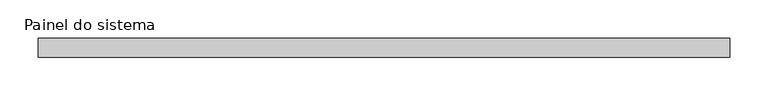
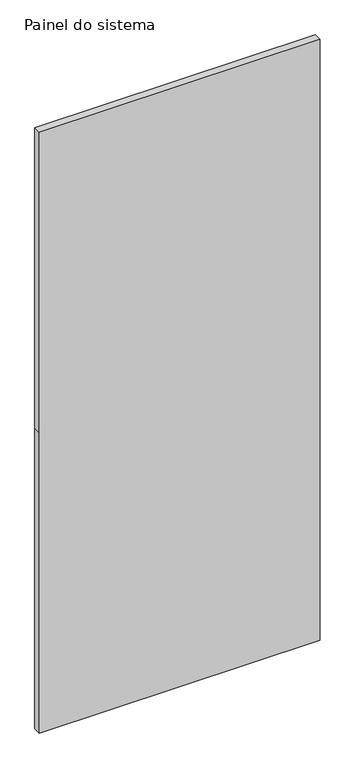
"""IFC4 building model written with IfcOpenShell, lengths in millimetres: plate geometry, Painel do sistema : Envidraçado."""

import ifcopenshell
import ifcopenshell.guid

model = None  # the IFC model being written
_history = None  # IfcOwnerHistory: only IFC2X3 demands one
_inside = {}  # id of a spatial element -> (the spatial element, [elements in it])
_under = {}  # id of a project, library or spatial element -> (it, [spatial elements below it])
_declared = {}  # id of a project -> (the project, [libraries it declares])
_typed = {}  # id of a type object -> (the type object, [elements of that type])
_made_of = {}  # id of a material, layer set ... -> (it, [elements and type objects made of it])


def new_model(schema):
    """Start an empty IFC model of exactly this schema.

    Asked for "IFC4X3", IfcOpenShell would pick the latest addendum, in which some entities
    have other attributes; the version numbers below select the first issue.
    IFC2X3 requires an IfcOwnerHistory on every rooted entity: one is made here for all.
    """
    global model, _history
    if schema == "IFC4X3":
        model = ifcopenshell.file(schema_version=(4, 3, 0, 0))
    else:
        model = ifcopenshell.file(schema=schema)
    _inside.clear()
    _under.clear()
    _declared.clear()
    _typed.clear()
    _made_of.clear()
    _history = None
    if model.schema == "IFC2X3":
        org = make("IfcOrganization", Name="unknown")
        user = make(
            "IfcPersonAndOrganization",
            ThePerson=make("IfcPerson", FamilyName="unknown"),
            TheOrganization=org,
        )
        app = make(
            "IfcApplication",
            ApplicationDeveloper=org,
            Version="unknown",
            ApplicationFullName="unknown",
            ApplicationIdentifier="unknown",
        )
        _history = make(
            "IfcOwnerHistory",
            OwningUser=user,
            OwningApplication=app,
            ChangeAction="ADDED",
            CreationDate=0,
        )
    return model


def make(cls, **values):
    """One entity of the class cls with the attributes given. An attribute that is None is left unset."""
    return model.create_entity(
        cls, **{name: value for name, value in values.items() if value is not None}
    )


def rooted(cls, **values):
    """An entity with a GlobalId (a new one), such as an element, a storey or a relation."""
    return make(cls, GlobalId=ifcopenshell.guid.new(), OwnerHistory=_history, **values)


def si_unit(unit_type, name, prefix=None):
    """IfcSIUnit, for example si_unit("LENGTHUNIT", "METRE", prefix="MILLI")."""
    return make("IfcSIUnit", UnitType=unit_type, Prefix=prefix, Name=name)


def assignment(units):
    """IfcUnitAssignment: the units of a project."""
    return None if units is None else make("IfcUnitAssignment", Units=units)


def point(xyz):
    """IfcCartesianPoint."""
    return None if xyz is None else make("IfcCartesianPoint", Coordinates=xyz)


def direction(xyz):
    """IfcDirection."""
    return None if xyz is None else make("IfcDirection", DirectionRatios=xyz)


def frame(location, z_axis=None, x_axis=None):
    """IfcAxis2Placement3D, a coordinate frame: its origin and axes. An axis left out is left unset."""
    return make(
        "IfcAxis2Placement3D",
        Location=point(location),
        Axis=direction(z_axis),
        RefDirection=direction(x_axis),
    )


def origin():
    """The frame at (0, 0, 0) with its axes left unset."""
    return frame((0.0, 0.0, 0.0))


def place(relative_to, where):
    """IfcLocalPlacement: puts the frame where relative to a parent placement (None: the world)."""
    return make(
        "IfcLocalPlacement", PlacementRelTo=relative_to, RelativePlacement=where
    )


def context(
    kind, dimensions, precision=None, world=None, true_north=None, identifier=None
):
    """IfcGeometricRepresentationContext, for example the 3D "Model" context."""
    return make(
        "IfcGeometricRepresentationContext",
        ContextIdentifier=identifier,
        ContextType=kind,
        CoordinateSpaceDimension=dimensions,
        Precision=precision,
        WorldCoordinateSystem=world,
        TrueNorth=true_north,
    )


def project(units=None, contexts=None):
    """IfcProject with its units and contexts."""
    return rooted(
        "IfcProject",
        Name="project",
        RepresentationContexts=contexts,
        UnitsInContext=assignment(units),
    )


def spatial(cls, under=None, at=None, **own):
    """A site, building, storey or space (cls), placed at a placement, below another one or the project."""
    s = rooted(cls, ObjectPlacement=at, **own)
    if under is not None:
        _under.setdefault(under.id(), (under, []))[1].append(s)
    return s


def polyline(points):
    """IfcPolyline through the points."""
    return make("IfcPolyline", Points=[point(p) for p in points])


def outline(outer, holes=None, kind="AREA"):
    """IfcArbitraryClosedProfileDef: a profile drawn as a closed curve; with holes, ...WithVoids."""
    if holes is None:
        return make("IfcArbitraryClosedProfileDef", ProfileType=kind, OuterCurve=outer)
    return make(
        "IfcArbitraryProfileDefWithVoids",
        ProfileType=kind,
        OuterCurve=outer,
        InnerCurves=holes,
    )


def extrude(swept, where, along, depth):
    """IfcExtrudedAreaSolid: the profile swept, set in the frame where, extruded along a direction by depth."""
    return make(
        "IfcExtrudedAreaSolid",
        SweptArea=swept,
        Position=where,
        ExtrudedDirection=direction(along),
        Depth=depth,
    )


def shape(context_of_items, identifier, shape_type, items):
    """IfcShapeRepresentation: the items that make up one representation, for example the "Body"."""
    return make(
        "IfcShapeRepresentation",
        ContextOfItems=context_of_items,
        RepresentationIdentifier=identifier,
        RepresentationType=shape_type,
        Items=items,
    )


def source(mapping_origin, context_of_items, identifier, shape_type, items):
    """IfcRepresentationMap: a shape defined once, which mapped items show again and again."""
    return make(
        "IfcRepresentationMap",
        MappingOrigin=mapping_origin,
        MappedRepresentation=shape(context_of_items, identifier, shape_type, items),
    )


def transform(
    local_origin,
    x_axis=None,
    y_axis=None,
    z_axis=None,
    scale=None,
    scale2=None,
    scale3=None,
    uniform=True,
):
    """IfcCartesianTransformationOperator3D, or its non-uniform kind. x_axis, y_axis, z_axis: its Axis1, 2, 3."""
    if uniform:
        return make(
            "IfcCartesianTransformationOperator3D",
            Axis1=direction(x_axis),
            Axis2=direction(y_axis),
            LocalOrigin=point(local_origin),
            Scale=scale,
            Axis3=direction(z_axis),
        )
    return make(
        "IfcCartesianTransformationOperator3DnonUniform",
        Axis1=direction(x_axis),
        Axis2=direction(y_axis),
        LocalOrigin=point(local_origin),
        Scale=scale,
        Axis3=direction(z_axis),
        Scale2=scale2,
        Scale3=scale3,
    )


def mapped(mapping_source, mapping_target):
    """IfcMappedItem: shows the shape of a source again, moved by a transform."""
    return make(
        "IfcMappedItem", MappingSource=mapping_source, MappingTarget=mapping_target
    )


def made_of(thing, what):
    """Note that an element or type object is made of a material, layer set ...; save() writes the relation."""
    if what is not None:
        _made_of.setdefault(what.id(), (what, []))[1].append(thing)
    return thing


def element(
    cls,
    number,
    at=None,
    inside=None,
    cuts=None,
    type_object=None,
    material=None,
    context=None,
    identifier="Body",
    shape_type=None,
    held_by="IfcProductDefinitionShape",
    body=None,
    shapes=None,
    **own,
):
    """One element of the class cls, such as IfcWall. Its Tag is "e" and its number.

    at: its placement. inside: the storey or other place that contains it. cuts: it is an
    opening in that element (IfcRelVoidsElement). A single representation is given by context,
    identifier, shape_type and body (its items); several are given by shapes. held_by: the class
    of the entity that holds the representations. save() writes the other relations.
    """
    e = rooted(cls, Tag="e%d" % number, ObjectPlacement=at, **own)
    if body is not None:
        shapes = [shape(context, identifier, shape_type, body)]
    if shapes is not None:
        e.Representation = make(held_by, Representations=shapes)
    if inside is not None:
        _inside.setdefault(inside.id(), (inside, []))[1].append(e)
    if cuts is not None:
        rooted(
            "IfcRelVoidsElement", RelatingBuildingElement=cuts, RelatedOpeningElement=e
        )
    if type_object is not None:
        _typed.setdefault(type_object.id(), (type_object, []))[1].append(e)
    return made_of(e, material)


def aggregate(whole, parts):
    """IfcRelAggregates: a whole, such as a stair, and the parts it consists of."""
    return rooted("IfcRelAggregates", RelatingObject=whole, RelatedObjects=parts)


def save(model, path):
    """Write the relations noted so far, then the file.

    IfcRelAggregates (storeys below a building ...), IfcRelContainedInSpatialStructure (elements
    in a storey), IfcRelDefinesByType, IfcRelAssociatesMaterial and IfcRelDeclares: one each for
    every whole, place, type object, material and project.
    """
    for whole, parts in _under.values():
        aggregate(whole, parts)
    for where, things in _inside.values():
        rooted(
            "IfcRelContainedInSpatialStructure",
            RelatedElements=things,
            RelatingStructure=where,
        )
    for kind, things in _typed.values():
        rooted("IfcRelDefinesByType", RelatedObjects=things, RelatingType=kind)
    for what, things in _made_of.values():
        rooted("IfcRelAssociatesMaterial", RelatedObjects=things, RelatingMaterial=what)
    for by, libraries in _declared.values():
        rooted("IfcRelDeclares", RelatingContext=by, RelatedDefinitions=libraries)
    model.write(path)


def painel_do_sistema_78d5b6fe(model_context):
    return source(origin(), model_context, "Body", "SweptSolid", [
        extrude(outline(polyline([(0.0, -453.0083333), (0.0, 453.0083333), (1025.0, 453.0083333), (2050.0, 453.0083333), (2050.0, -453.0083333), (1025.0, -453.0083333), (0.0, -453.0083333)])), frame((0.0, 24.5, 0.0), z_axis=(0.0, 1.0, 0.0), x_axis=(0.0, 0.0, 1.0)), (0.0, 0.0, 1.0), 25.0),
    ])


if __name__ == "__main__":
    model = new_model("IFC4")
    model_context = context("Model", 3, world=origin())
    ifc_project = project(units=[si_unit("LENGTHUNIT", "METRE", prefix="MILLI")], contexts=[model_context])
    site = spatial("IfcSite", under=ifc_project)
    building = spatial("IfcBuilding", under=site)
    placement = place(None, origin())
    painel_do_sistema_shape = painel_do_sistema_78d5b6fe(model_context)
    element("IfcPlate", 1, ObjectType="Painel do sistema : Envidraçado", at=placement, inside=building, context=model_context, shape_type="MappedRepresentation", body=[
        mapped(painel_do_sistema_shape, transform((0.0, 0.0, 0.0), x_axis=(1.0, 0.0, 0.0), y_axis=(0.0, 1.0, 0.0), z_axis=(0.0, 0.0, 1.0))),
    ])
    save(model, "model.ifc")

# Revit data of these elements
# Type "Painel do sistema : Envidraçado"
#   Construction Type Id = "GSP4R"
#   Analytic Construction = "Vidraça única Pilkington 1/8 pol"
#   Visual Light Transmittance = 0.9
#   Solar Heat Gain Coefficient = 0.86
#   Heat Transfer Coefficient (U) = 6.7069 W/(m²·K)
# Element 1 (IfcPlate, "Painel do sistema : Envidraçado")
#   Materials on its faces: ".VIDRO GENÉRICO"
# Materials
#   ".VIDRO GENÉRICO": class ".CC_VIDRO", colour RGB 0 128 192, transparency 0.9, Description = "Vidro comum", Cost = 0
